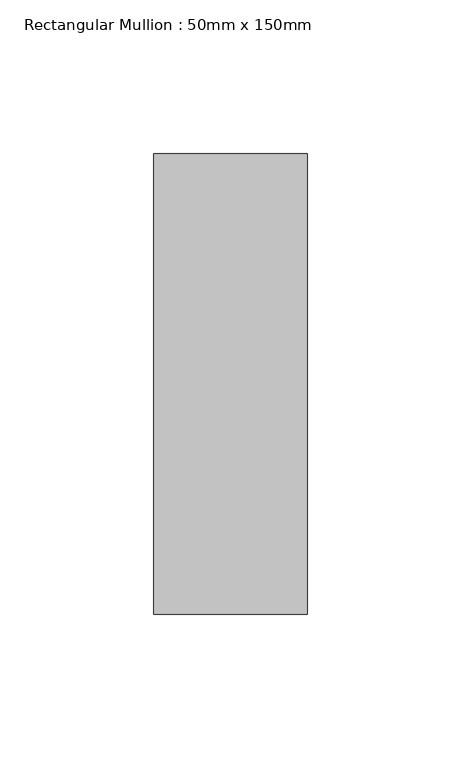
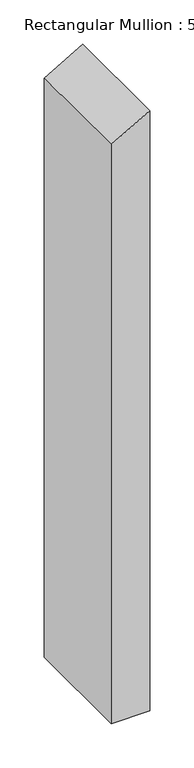
"""IFC4 building model written with IfcOpenShell, lengths in millimetres: member geometry, Rectangular Mullion : 50mm x 150mm."""

from ifc_helpers import new_model, si_unit, frame, origin, place, context, project, spatial, polyline, outline, extrude, source, transform, mapped, element, save


def rectangular_mullion_50mm_x_150mm_892e7b11(model_context):
    return source(origin(), model_context, "Body", "SweptSolid", [
        extrude(outline(polyline([(0.0, 0.0), (-28.8675135, -50.0), (-824.7860988, -50.0), (-824.7860988, 0.0), (0.0, 0.0)])), frame((0.0, -75.0, 0.0), z_axis=(0.0, 1.0, 0.0), x_axis=(0.0, 0.0, 1.0)), (0.0, 0.0, 1.0), 150.0),
    ])


if __name__ == "__main__":
    model = new_model("IFC4")
    model_context = context("Model", 3, world=origin())
    ifc_project = project(units=[si_unit("LENGTHUNIT", "METRE", prefix="MILLI")], contexts=[model_context])
    site = spatial("IfcSite", under=ifc_project)
    building = spatial("IfcBuilding", under=site)
    placement = place(None, origin())
    rectangular_mullion_50mm_x_150mm_shape = rectangular_mullion_50mm_x_150mm_892e7b11(model_context)
    element("IfcMember", 1, ObjectType="Rectangular Mullion : 50mm x 150mm", at=placement, inside=building, context=model_context, shape_type="MappedRepresentation", body=[
        mapped(rectangular_mullion_50mm_x_150mm_shape, transform((0.0, 0.0, 0.0), x_axis=(1.0, 0.0, 0.0), y_axis=(0.0, 1.0, 0.0), z_axis=(0.0, 0.0, 1.0))),
    ])
    save(model, "model.ifc")

# Revit data of these elements
# Type "Rectangular Mullion : 50mm x 150mm"
#   built-in parameter 1007304 = 0.492126 (stored number, unit not read)
#   built-in parameter 1007301 = 0.082021 (stored number, unit not read)
#   built-in parameter 1007300 = 0.082021 (stored number, unit not read)
# Element 1 (IfcMember, "Rectangular Mullion : 50mm x 150mm")
#   Materials on its faces: "Aluminum"
# Materials
#   "Aluminum": class "Metal", colour RGB 247 247 247, transparency 0, Description = "Aluminum 6061", Cost = 0
